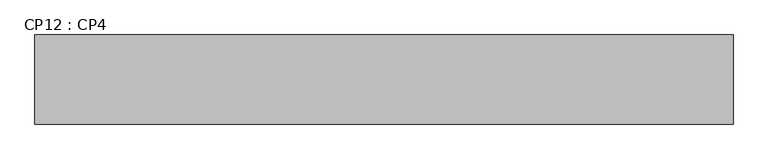
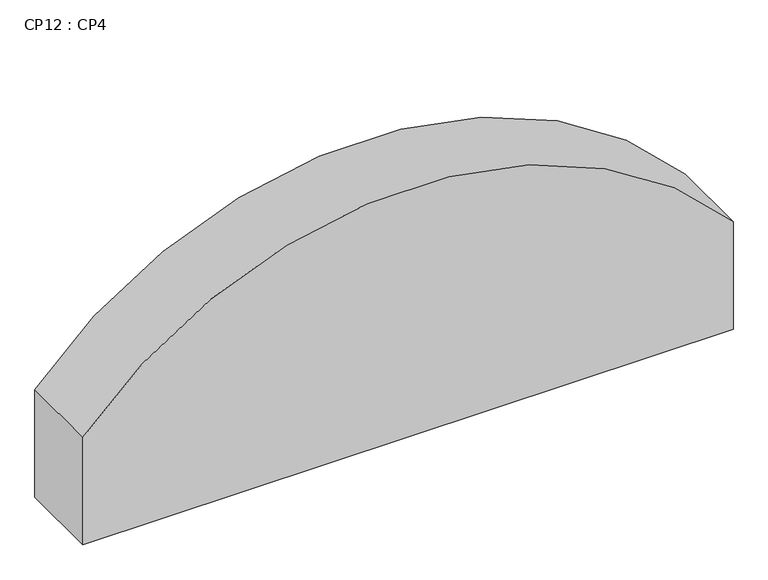
"""IFC4 building model written with IfcOpenShell, lengths in millimetres: beam geometry, CP12 : CP4."""

from ifc_helpers import new_model, si_unit, frame, origin, place, context, project, spatial, circle_curve, source, transform, mapped, element, save
from ifc_brep_helpers import plane_surface, cylinder_surface, advanced_brep


def cp12_cp4_946f0f9f(model_context):
    return source(origin(), model_context, "Body", "AdvancedBrep", [
        advanced_brep(
        [(30483.2245515, 499.6999991, 14620.0), (35183.2245514, 499.6999991, 14620.0), (35183.2245494, 499.6999991, 13800.0), (30483.2245488, 499.6999991, 13800.0), (35183.2245514, -100.2551788, 14620.0), (30483.2245515, -100.2551788, 14620.0), (30483.2245488, -100.2551788, 13800.0), (35183.2245494, -100.2551788, 13800.0)],
        [
            (0, 1, circle_curve(frame((32833.2245514, 499.6999991, 12603.2870371), z_axis=(0.0, 1.0, 0.0), x_axis=(0.0, 0.0, -1.0)), 3096.7129629)),
            (1, 2),
            (2, 3),
            (3, 0),
            (4, 5, circle_curve(frame((32833.2245514, -100.2551788, 12603.2870371), z_axis=(0.0, -1.0, 0.0), x_axis=(0.0, 0.0, -1.0)), 3096.7129629)),
            (5, 6),
            (6, 7),
            (7, 4),
            (6, 3),
            (2, 7),
            (0, 5),
            (4, 1),
        ],
        [
            plane_surface(frame((32833.2245514, 499.6999991, 9323.3898307), z_axis=(0.0, 1.0, 0.0), x_axis=(-1.0, 0.0, 0.0))),
            plane_surface(frame((32833.2245514, -100.2551788, 9323.3898307), z_axis=(0.0, -1.0, 0.0), x_axis=(1.0, 0.0, 0.0))),
            plane_surface(frame((35333.2245514, 499.6999991, 13800.0), z_axis=(0.0, 0.0, -1.0), x_axis=(0.0, -1.0, 0.0))),
            cylinder_surface(frame((32833.2245514, 20099.7448193, 12603.2870371), z_axis=(0.0, 1.0, 0.0), x_axis=(0.0, 0.0, -1.0)), 3096.7129629),
            plane_surface(frame((30483.2245488, 18587.0448193, 14620.0), z_axis=(-1.0, 0.0, 0.0), x_axis=(0.0, -1.0, 0.0))),
            plane_surface(frame((35183.2245494, 18587.0448193, 13800.0), z_axis=(1.0, 0.0, 0.0), x_axis=(0.0, -1.0, 0.0))),
        ],
        [
            (0, [[1, 2, 3, 4]]),
            (1, [[5, 6, 7, 8]]),
            (2, [[9, -3, 10, -7]]),
            (3, [[-1, 11, -5, 12]]),
            (4, [[-4, -9, -6, -11]]),
            (5, [[-2, -12, -8, -10]]),
        ],
    ),
    ])


if __name__ == "__main__":
    model = new_model("IFC4")
    model_context = context("Model", 3, world=origin())
    ifc_project = project(units=[si_unit("LENGTHUNIT", "METRE", prefix="MILLI")], contexts=[model_context])
    site = spatial("IfcSite", under=ifc_project)
    building = spatial("IfcBuilding", under=site)
    placement = place(None, origin())
    cp12_cp4_shape = cp12_cp4_946f0f9f(model_context)
    element("IfcBeam", 1, ObjectType="CP12 : CP4", at=placement, inside=building, context=model_context, shape_type="MappedRepresentation", body=[
        mapped(cp12_cp4_shape, transform((0.0, 0.0, 0.0), x_axis=(1.0, 0.0, 0.0), y_axis=(0.0, 1.0, 0.0), z_axis=(0.0, 0.0, 1.0))),
    ])
    save(model, "model.ifc")
